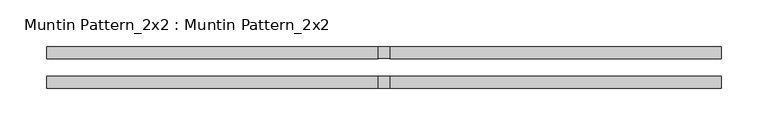
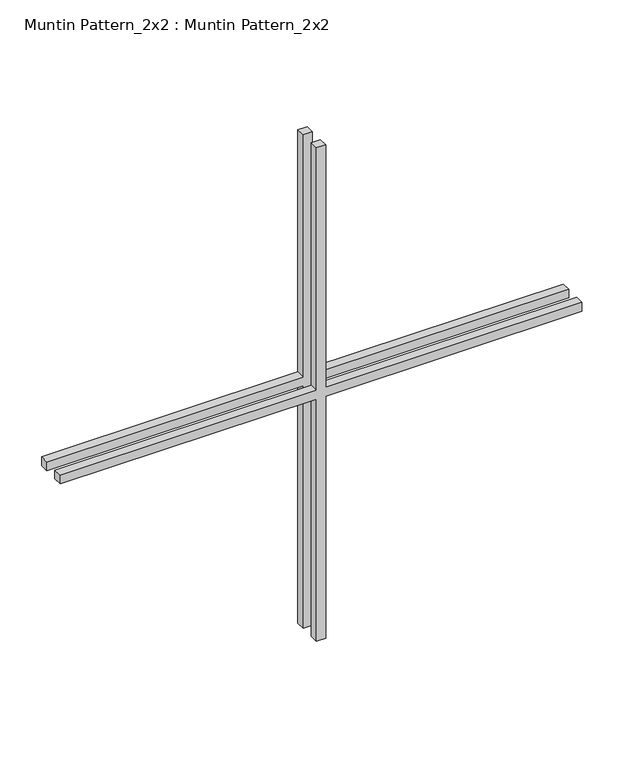
"""IFC4 building model written with IfcOpenShell, lengths in millimetres: proxy geometry, Muntin Pattern_2x2 : Muntin Pattern_2x2."""

from ifc_helpers import new_model, si_unit, frame, origin, place, context, project, spatial, polyline, outline, extrude, source, transform, mapped, element, save


def muntin_pattern_2x2_muntin_pattern_2x2_001fa0c9(model_context):
    return source(origin(), model_context, "Body", "SweptSolid", [
        extrude(outline(polyline([(368.3, -6.35), (368.3, -361.95), (355.6, -361.95), (355.6, -6.35), (0.0, -6.35), (0.0, 6.35), (355.6, 6.35), (355.6, 361.95), (368.3, 361.95), (368.3, 6.35), (723.9, 6.35), (723.9, -6.35), (368.3, -6.35)])), frame((0.0, 9.525, 0.0), z_axis=(0.0, 1.0, 0.0), x_axis=(0.0, 0.0, 1.0)), (0.0, 0.0, 1.0), 12.7),
        extrude(outline(polyline([(368.3, -6.35), (368.3, -361.95), (355.6, -361.95), (355.6, -6.35), (0.0, -6.35), (0.0, 6.35), (355.6, 6.35), (355.6, 361.95), (368.3, 361.95), (368.3, 6.35), (723.9, 6.35), (723.9, -6.35), (368.3, -6.35)])), frame((0.0, -22.225, 0.0), z_axis=(0.0, 1.0, 0.0), x_axis=(0.0, 0.0, 1.0)), (0.0, 0.0, 1.0), 12.7),
    ])


if __name__ == "__main__":
    model = new_model("IFC4")
    model_context = context("Model", 3, world=origin())
    ifc_project = project(units=[si_unit("LENGTHUNIT", "METRE", prefix="MILLI")], contexts=[model_context])
    site = spatial("IfcSite", under=ifc_project)
    building = spatial("IfcBuilding", under=site)
    placement = place(None, origin())
    muntin_pattern_2x2_muntin_pattern_2x2_shape = muntin_pattern_2x2_muntin_pattern_2x2_001fa0c9(model_context)
    element("IfcBuildingElementProxy", 1, Name="Muntin Pattern_2x2 : Muntin Pattern_2x2", ObjectType="Muntin Pattern_2x2 : Muntin Pattern_2x2", at=placement, inside=building, context=model_context, shape_type="MappedRepresentation", body=[
        mapped(muntin_pattern_2x2_muntin_pattern_2x2_shape, transform((0.0, 0.0, 0.0), x_axis=(1.0, 0.0, 0.0), y_axis=(0.0, 1.0, 0.0), z_axis=(0.0, 0.0, 1.0))),
    ])
    save(model, "model.ifc")

# Revit data of these elements
# Type "Muntin Pattern_2x2 : Muntin Pattern_2x2"
#   Width [instance default] = 4' - 0"
#   Thickness = 0' - 0 1/2"
#   Height [instance default] = 4' - 0"
#   Distance = 0' - 0 3/4"
#   Interior Material [instance default] = none
#   Exterior Material [instance default] = none
# Element 1 (IfcBuildingElementProxy, "Muntin Pattern_2x2 : Muntin Pattern_2x2")
#   Width = 2' - 4 1/2"
#   Height = 2' - 4 1/2"
#   Interior Material = 1X WOOD COMPOSITE TRIM
#   Exterior Material = 1X WOOD COMPOSITE TRIM
#   Materials on its faces: "1X WOOD COMPOSITE TRIM"
# Materials
#   "1X WOOD COMPOSITE TRIM": class "Generic", colour RGB 88 61 61, transparency 0, Cost = 0
